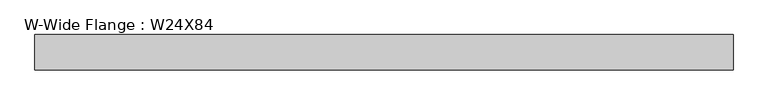
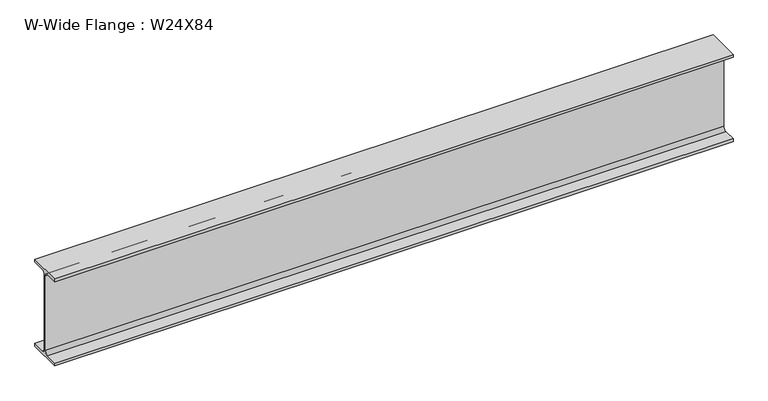
"""IFC4 building model written with IfcOpenShell, lengths in millimetres: beam geometry, W-Wide Flange : W24X84."""

from ifc_helpers import new_model, si_unit, point, frame, frame_2d, origin, place, context, project, spatial, polyline, circle_curve, trimmed, segment, composite_curve, outline, extrude, source, transform, mapped, element, save


def w_wide_flange_w24x84_4409fa3f(model_context):
    return source(origin(), model_context, "Body", "SweptSolid", [
        extrude(outline(composite_curve([segment(polyline([(114.554, -286.512), (114.554, -306.07), (-114.554, -306.07), (-114.554, -286.512), (-29.2735, -286.512)]), True, "CONTINUOUS"), segment(trimmed(circle_curve(frame_2d((-29.2735, -263.2075)), 23.3045), [point((-29.2735, -286.512))], [point((-5.969, -263.2075))], True, "CARTESIAN"), True, "CONTINUOUS"), segment(polyline([(-5.969, -263.2075), (-5.969, 263.2075)]), True, "CONTINUOUS"), segment(trimmed(circle_curve(frame_2d((-29.2735, 263.2075)), 23.3045), [point((-5.969, 263.2075))], [point((-29.2735, 286.512))], True, "CARTESIAN"), True, "CONTINUOUS"), segment(polyline([(-29.2735, 286.512), (-114.554, 286.512), (-114.554, 306.07), (114.554, 306.07), (114.554, 286.512), (29.2735, 286.512)]), True, "CONTINUOUS"), segment(trimmed(circle_curve(frame_2d((29.2735, 263.2075)), 23.3045), [point((29.2735, 286.512))], [point((5.969, 263.2075))], True, "CARTESIAN"), True, "CONTINUOUS"), segment(polyline([(5.969, 263.2075), (5.969, -263.2075)]), True, "CONTINUOUS"), segment(trimmed(circle_curve(frame_2d((29.2735, -263.2075)), 23.3045), [point((5.969, -263.2075))], [point((29.2735, -286.512))], True, "CARTESIAN"), True, "CONTINUOUS"), segment(polyline([(29.2735, -286.512), (114.554, -286.512)]), True, "CONTINUOUS")], self_intersect=False)), frame((-2263.3037109, 0.0, 0.0), z_axis=(1.0, 0.0, 0.0), x_axis=(0.0, 1.0, 0.0)), (0.0, 0.0, 1.0), 4513.1632812),
    ])


if __name__ == "__main__":
    model = new_model("IFC4")
    model_context = context("Model", 3, world=origin())
    ifc_project = project(units=[si_unit("LENGTHUNIT", "METRE", prefix="MILLI")], contexts=[model_context])
    site = spatial("IfcSite", under=ifc_project)
    building = spatial("IfcBuilding", under=site)
    placement = place(None, origin())
    w_wide_flange_w24x84_shape = w_wide_flange_w24x84_4409fa3f(model_context)
    element("IfcBeam", 1, ObjectType="W-Wide Flange : W24X84", at=placement, inside=building, context=model_context, shape_type="MappedRepresentation", body=[
        mapped(w_wide_flange_w24x84_shape, transform((0.0, 0.0, 0.0), x_axis=(1.0, 0.0, 0.0), y_axis=(0.0, 1.0, 0.0), z_axis=(0.0, 0.0, 1.0))),
    ])
    save(model, "model.ifc")

# Revit data of these elements
# Type "W-Wide Flange : W24X84"
#   Assembly Code = "B10"
#   W = 84
#   Length [instance default] = 1524 mm
#   bf = 229.108 mm
#   d = 612.14 mm
#   k = 42.863 mm
#   k2 = 23.305 mm
#   tf = 19.558 mm
#   tw = 11.938 mm
#   A = 0.0159355 m²
#   Structural Material [instance default] = Steel ASTM A992
# Element 1 (IfcBeam, "W-Wide Flange : W24X84")
#   Structural Material = Aluminum, Anodized Red
#   Materials on its faces: "Aluminum, Anodized Red"
# Materials
#   "Steel ASTM A992": class "Metal", colour RGB 128 0 0, transparency 0, Description = "Structural steel 50ksi", Cost = 0
#   "Aluminum, Anodized Red": class "Metal", colour RGB 120 120 120, transparency 0, Description = "Anodized aluminum, red", Cost = 0
